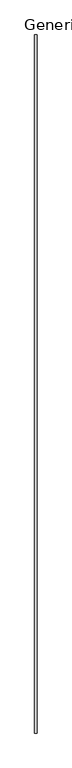
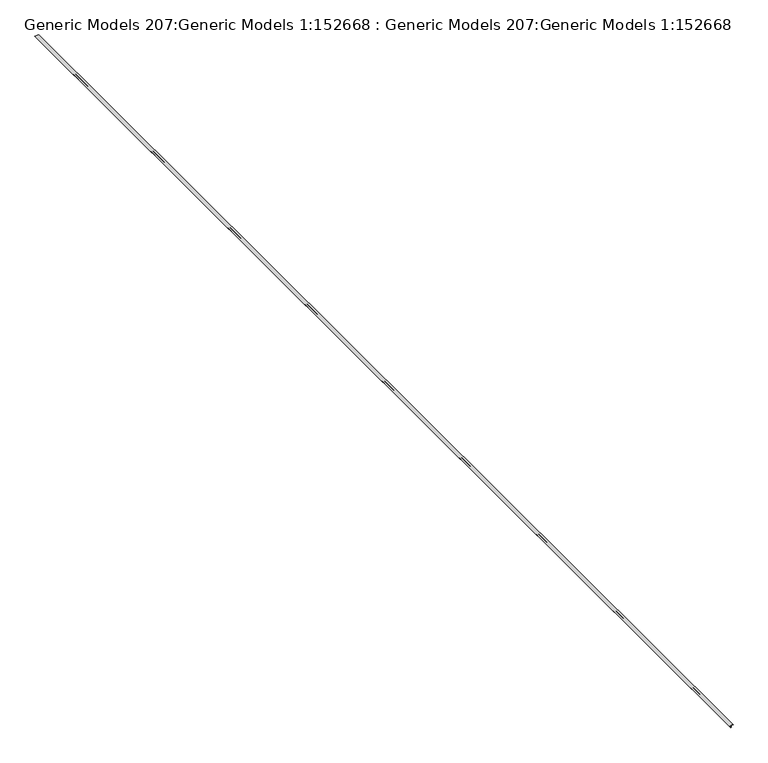
"""IFC4 building model written with IfcOpenShell, lengths in millimetres: proxy geometry, Generic Models 207:Generic Models 1:152668 : Generic Models 207:Generic Models 1:152668."""

from ifc_helpers import new_model, si_unit, frame, origin, place, context, project, spatial, polyline, outline, extrude, source, transform, mapped, element, save


def generic_models_207_generic_models_1_152668_generic_models_ba32aa02(model_context):
    return source(origin(), model_context, "Body", "SweptSolid", [
        extrude(outline(polyline([(3065.78, -8197.971787), (3067.05, -8197.971787), (3067.05, -8237.341787), (3065.78, -8237.341787), (3065.78, -8218.291787), (3046.095, -8218.291787), (3046.095, -8221.771587), (3044.825, -8221.771587), (3044.825, -8217.021787), (3065.78, -8217.021787), (3065.78, -8197.971787)])), frame((0.0, -273.9974793, 0.0), z_axis=(0.0, 1.0, 0.0), x_axis=(0.0, 0.0, 1.0)), (0.0, 0.0, 1.0), 12446.0),
    ])


if __name__ == "__main__":
    model = new_model("IFC4")
    model_context = context("Model", 3, world=origin())
    ifc_project = project(units=[si_unit("LENGTHUNIT", "METRE", prefix="MILLI")], contexts=[model_context])
    site = spatial("IfcSite", under=ifc_project)
    building = spatial("IfcBuilding", under=site)
    placement = place(None, origin())
    generic_models_207_generic_models_1_152668_generic_models_shape = generic_models_207_generic_models_1_152668_generic_models_ba32aa02(model_context)
    element("IfcBuildingElementProxy", 1, Name="Generic Models 207:Generic Models 1:152668 : Generic Models 207:Generic Models 1:152668", ObjectType="Generic Models 207:Generic Models 1:152668 : Generic Models 207:Generic Models 1:152668", at=placement, inside=building, context=model_context, shape_type="MappedRepresentation", body=[
        mapped(generic_models_207_generic_models_1_152668_generic_models_shape, transform((0.0, 0.0, 0.0), x_axis=(1.0, 0.0, 0.0), y_axis=(0.0, 1.0, 0.0), z_axis=(0.0, 0.0, 1.0))),
    ])
    save(model, "model.ifc")

# Revit data of these elements
# Type "Generic Models 207:Generic Models 1:152668 : Generic Models 207:Generic Models 1:152668"
#   NameOverride = "Generic Models 207:Generic Models 1:152668"
#   ObjectTypeOverride = "Generic Models 207:Generic Models 1"
#   Reference = "Generic Models 1"
#   Category = "Generic Models"
#   Tag = "152668"
# Element 1 (IfcBuildingElementProxy, "Generic Models 207:Generic Models 1:152668 : Generic Models 207:Generic Models 1:152668")
#   Materials on its faces: "_16 GA. COPPER VENTED REVEAL MOLDING 6770"
# Materials
#   "_16 GA. COPPER VENTED REVEAL MOLDING 6770": class "Unassigned", colour RGB 253 192 103, transparency 0
